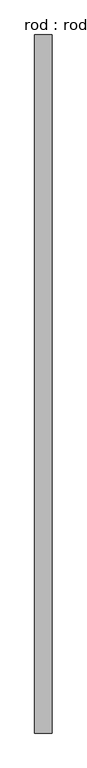
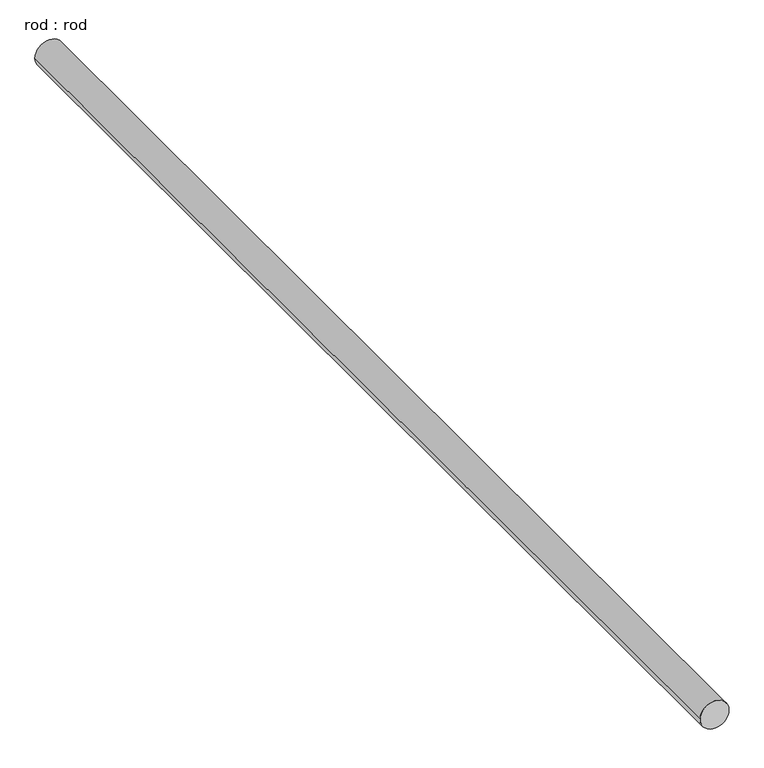
"""IFC4 building model written with IfcOpenShell, lengths in millimetres: proxy geometry, rod : rod."""

from ifc_helpers import new_model, si_unit, point, frame, frame_2d, origin, place, context, project, spatial, circle_curve, trimmed, segment, composite_curve, outline, extrude, source, transform, mapped, element, save


def rod_rod_0ebd8051(model_context):
    return source(origin(), model_context, "Body", "SweptSolid", [
        extrude(outline(composite_curve([segment(trimmed(circle_curve(frame_2d((0.0108462, 0.0)), 200.0), [point((0.0108462, 200.0))], [point((0.0108462, -200.0))], False, "CARTESIAN"), True, "CONTINUOUS"), segment(trimmed(circle_curve(frame_2d((0.0108462, 0.0)), 200.0), [point((0.0108462, -200.0))], [point((0.0108462, 200.0))], False, "CARTESIAN"), True, "CONTINUOUS")], self_intersect=False)), frame((0.0, -3883.7995139, 0.0), z_axis=(0.0, 1.0, 0.0), x_axis=(0.0, 0.0, 1.0)), (0.0, 0.0, 1.0), 15953.0562585),
    ])


if __name__ == "__main__":
    model = new_model("IFC4")
    model_context = context("Model", 3, world=origin())
    ifc_project = project(units=[si_unit("LENGTHUNIT", "METRE", prefix="MILLI")], contexts=[model_context])
    site = spatial("IfcSite", under=ifc_project)
    building = spatial("IfcBuilding", under=site)
    placement = place(None, origin())
    rod_rod_shape = rod_rod_0ebd8051(model_context)
    element("IfcBuildingElementProxy", 1, Name="rod : rod", ObjectType="rod : rod", at=placement, inside=building, context=model_context, shape_type="MappedRepresentation", body=[
        mapped(rod_rod_shape, transform((0.0, 0.0, 0.0), x_axis=(1.0, 0.0, 0.0), y_axis=(0.0, 1.0, 0.0), z_axis=(0.0, 0.0, 1.0))),
    ])
    save(model, "model.ifc")

# Revit data of these elements
# Type "rod : rod"
#   Default Elevation = 0
